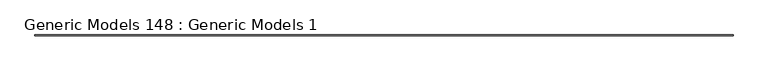
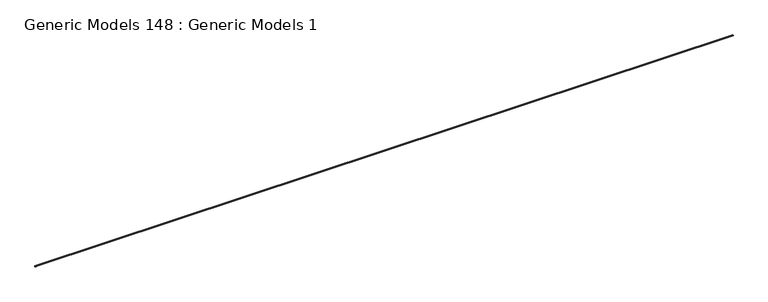
"""IFC4 building model written with IfcOpenShell, lengths in millimetres: proxy geometry, Generic Models 148 : Generic Models 1."""

import ifcopenshell
import ifcopenshell.guid

model = None  # the IFC model being written
_history = None  # IfcOwnerHistory: only IFC2X3 demands one
_inside = {}  # id of a spatial element -> (the spatial element, [elements in it])
_under = {}  # id of a project, library or spatial element -> (it, [spatial elements below it])
_declared = {}  # id of a project -> (the project, [libraries it declares])
_typed = {}  # id of a type object -> (the type object, [elements of that type])
_made_of = {}  # id of a material, layer set ... -> (it, [elements and type objects made of it])


def new_model(schema):
    """Start an empty IFC model of exactly this schema.

    Asked for "IFC4X3", IfcOpenShell would pick the latest addendum, in which some entities
    have other attributes; the version numbers below select the first issue.
    IFC2X3 requires an IfcOwnerHistory on every rooted entity: one is made here for all.
    """
    global model, _history
    if schema == "IFC4X3":
        model = ifcopenshell.file(schema_version=(4, 3, 0, 0))
    else:
        model = ifcopenshell.file(schema=schema)
    _inside.clear()
    _under.clear()
    _declared.clear()
    _typed.clear()
    _made_of.clear()
    _history = None
    if model.schema == "IFC2X3":
        org = make("IfcOrganization", Name="unknown")
        user = make(
            "IfcPersonAndOrganization",
            ThePerson=make("IfcPerson", FamilyName="unknown"),
            TheOrganization=org,
        )
        app = make(
            "IfcApplication",
            ApplicationDeveloper=org,
            Version="unknown",
            ApplicationFullName="unknown",
            ApplicationIdentifier="unknown",
        )
        _history = make(
            "IfcOwnerHistory",
            OwningUser=user,
            OwningApplication=app,
            ChangeAction="ADDED",
            CreationDate=0,
        )
    return model


def make(cls, **values):
    """One entity of the class cls with the attributes given. An attribute that is None is left unset."""
    return model.create_entity(
        cls, **{name: value for name, value in values.items() if value is not None}
    )


def rooted(cls, **values):
    """An entity with a GlobalId (a new one), such as an element, a storey or a relation."""
    return make(cls, GlobalId=ifcopenshell.guid.new(), OwnerHistory=_history, **values)


def si_unit(unit_type, name, prefix=None):
    """IfcSIUnit, for example si_unit("LENGTHUNIT", "METRE", prefix="MILLI")."""
    return make("IfcSIUnit", UnitType=unit_type, Prefix=prefix, Name=name)


def assignment(units):
    """IfcUnitAssignment: the units of a project."""
    return None if units is None else make("IfcUnitAssignment", Units=units)


def point(xyz):
    """IfcCartesianPoint."""
    return None if xyz is None else make("IfcCartesianPoint", Coordinates=xyz)


def direction(xyz):
    """IfcDirection."""
    return None if xyz is None else make("IfcDirection", DirectionRatios=xyz)


def frame(location, z_axis=None, x_axis=None):
    """IfcAxis2Placement3D, a coordinate frame: its origin and axes. An axis left out is left unset."""
    return make(
        "IfcAxis2Placement3D",
        Location=point(location),
        Axis=direction(z_axis),
        RefDirection=direction(x_axis),
    )


def frame_2d(location, x_axis=None):
    """IfcAxis2Placement2D, a coordinate frame in the plane: its origin and x axis."""
    return make(
        "IfcAxis2Placement2D", Location=point(location), RefDirection=direction(x_axis)
    )


def origin():
    """The frame at (0, 0, 0) with its axes left unset."""
    return frame((0.0, 0.0, 0.0))


def place(relative_to, where):
    """IfcLocalPlacement: puts the frame where relative to a parent placement (None: the world)."""
    return make(
        "IfcLocalPlacement", PlacementRelTo=relative_to, RelativePlacement=where
    )


def context(
    kind, dimensions, precision=None, world=None, true_north=None, identifier=None
):
    """IfcGeometricRepresentationContext, for example the 3D "Model" context."""
    return make(
        "IfcGeometricRepresentationContext",
        ContextIdentifier=identifier,
        ContextType=kind,
        CoordinateSpaceDimension=dimensions,
        Precision=precision,
        WorldCoordinateSystem=world,
        TrueNorth=true_north,
    )


def project(units=None, contexts=None):
    """IfcProject with its units and contexts."""
    return rooted(
        "IfcProject",
        Name="project",
        RepresentationContexts=contexts,
        UnitsInContext=assignment(units),
    )


def spatial(cls, under=None, at=None, **own):
    """A site, building, storey or space (cls), placed at a placement, below another one or the project."""
    s = rooted(cls, ObjectPlacement=at, **own)
    if under is not None:
        _under.setdefault(under.id(), (under, []))[1].append(s)
    return s


def polyline(points):
    """IfcPolyline through the points."""
    return make("IfcPolyline", Points=[point(p) for p in points])


def circle_curve(where, radius):
    """IfcCircle in the frame where."""
    return make("IfcCircle", Position=where, Radius=radius)


def trimmed(basis, trim1, trim2, sense, master):
    """IfcTrimmedCurve: the piece of a basis curve between two trims."""
    return make(
        "IfcTrimmedCurve",
        BasisCurve=basis,
        Trim1=trim1,
        Trim2=trim2,
        SenseAgreement=sense,
        MasterRepresentation=master,
    )


def segment(curve, same_sense, transition):
    """IfcCompositeCurveSegment."""
    return make(
        "IfcCompositeCurveSegment",
        Transition=transition,
        SameSense=same_sense,
        ParentCurve=curve,
    )


def composite_curve(segments, self_intersect=None):
    """IfcCompositeCurve: segments joined end to end."""
    return make("IfcCompositeCurve", Segments=segments, SelfIntersect=self_intersect)


def outline(outer, holes=None, kind="AREA"):
    """IfcArbitraryClosedProfileDef: a profile drawn as a closed curve; with holes, ...WithVoids."""
    if holes is None:
        return make("IfcArbitraryClosedProfileDef", ProfileType=kind, OuterCurve=outer)
    return make(
        "IfcArbitraryProfileDefWithVoids",
        ProfileType=kind,
        OuterCurve=outer,
        InnerCurves=holes,
    )


def extrude(swept, where, along, depth):
    """IfcExtrudedAreaSolid: the profile swept, set in the frame where, extruded along a direction by depth."""
    return make(
        "IfcExtrudedAreaSolid",
        SweptArea=swept,
        Position=where,
        ExtrudedDirection=direction(along),
        Depth=depth,
    )


def shape(context_of_items, identifier, shape_type, items):
    """IfcShapeRepresentation: the items that make up one representation, for example the "Body"."""
    return make(
        "IfcShapeRepresentation",
        ContextOfItems=context_of_items,
        RepresentationIdentifier=identifier,
        RepresentationType=shape_type,
        Items=items,
    )


def source(mapping_origin, context_of_items, identifier, shape_type, items):
    """IfcRepresentationMap: a shape defined once, which mapped items show again and again."""
    return make(
        "IfcRepresentationMap",
        MappingOrigin=mapping_origin,
        MappedRepresentation=shape(context_of_items, identifier, shape_type, items),
    )


def transform(
    local_origin,
    x_axis=None,
    y_axis=None,
    z_axis=None,
    scale=None,
    scale2=None,
    scale3=None,
    uniform=True,
):
    """IfcCartesianTransformationOperator3D, or its non-uniform kind. x_axis, y_axis, z_axis: its Axis1, 2, 3."""
    if uniform:
        return make(
            "IfcCartesianTransformationOperator3D",
            Axis1=direction(x_axis),
            Axis2=direction(y_axis),
            LocalOrigin=point(local_origin),
            Scale=scale,
            Axis3=direction(z_axis),
        )
    return make(
        "IfcCartesianTransformationOperator3DnonUniform",
        Axis1=direction(x_axis),
        Axis2=direction(y_axis),
        LocalOrigin=point(local_origin),
        Scale=scale,
        Axis3=direction(z_axis),
        Scale2=scale2,
        Scale3=scale3,
    )


def mapped(mapping_source, mapping_target):
    """IfcMappedItem: shows the shape of a source again, moved by a transform."""
    return make(
        "IfcMappedItem", MappingSource=mapping_source, MappingTarget=mapping_target
    )


def made_of(thing, what):
    """Note that an element or type object is made of a material, layer set ...; save() writes the relation."""
    if what is not None:
        _made_of.setdefault(what.id(), (what, []))[1].append(thing)
    return thing


def element(
    cls,
    number,
    at=None,
    inside=None,
    cuts=None,
    type_object=None,
    material=None,
    context=None,
    identifier="Body",
    shape_type=None,
    held_by="IfcProductDefinitionShape",
    body=None,
    shapes=None,
    **own,
):
    """One element of the class cls, such as IfcWall. Its Tag is "e" and its number.

    at: its placement. inside: the storey or other place that contains it. cuts: it is an
    opening in that element (IfcRelVoidsElement). A single representation is given by context,
    identifier, shape_type and body (its items); several are given by shapes. held_by: the class
    of the entity that holds the representations. save() writes the other relations.
    """
    e = rooted(cls, Tag="e%d" % number, ObjectPlacement=at, **own)
    if body is not None:
        shapes = [shape(context, identifier, shape_type, body)]
    if shapes is not None:
        e.Representation = make(held_by, Representations=shapes)
    if inside is not None:
        _inside.setdefault(inside.id(), (inside, []))[1].append(e)
    if cuts is not None:
        rooted(
            "IfcRelVoidsElement", RelatingBuildingElement=cuts, RelatedOpeningElement=e
        )
    if type_object is not None:
        _typed.setdefault(type_object.id(), (type_object, []))[1].append(e)
    return made_of(e, material)


def aggregate(whole, parts):
    """IfcRelAggregates: a whole, such as a stair, and the parts it consists of."""
    return rooted("IfcRelAggregates", RelatingObject=whole, RelatedObjects=parts)


def save(model, path):
    """Write the relations noted so far, then the file.

    IfcRelAggregates (storeys below a building ...), IfcRelContainedInSpatialStructure (elements
    in a storey), IfcRelDefinesByType, IfcRelAssociatesMaterial and IfcRelDeclares: one each for
    every whole, place, type object, material and project.
    """
    for whole, parts in _under.values():
        aggregate(whole, parts)
    for where, things in _inside.values():
        rooted(
            "IfcRelContainedInSpatialStructure",
            RelatedElements=things,
            RelatingStructure=where,
        )
    for kind, things in _typed.values():
        rooted("IfcRelDefinesByType", RelatedObjects=things, RelatingType=kind)
    for what, things in _made_of.values():
        rooted("IfcRelAssociatesMaterial", RelatedObjects=things, RelatingMaterial=what)
    for by, libraries in _declared.values():
        rooted("IfcRelDeclares", RelatingContext=by, RelatedDefinitions=libraries)
    model.write(path)


def generic_models_148_generic_models_1_1e1312a9(model_context):
    return source(origin(), model_context, "Body", "SweptSolid", [
        extrude(outline(composite_curve([segment(trimmed(circle_curve(frame_2d((7062.6754549, 123920.3246075)), 8.620055), [point((7056.3254549, 123914.4951265))], [point((7069.0254549, 123914.4951265))], True, "CARTESIAN"), True, "CONTINUOUS"), segment(polyline([(7069.0254549, 123914.4951265), (7069.0254549, 123904.9701265)]), True, "CONTINUOUS"), segment(trimmed(circle_curve(frame_2d((7062.6754549, 123910.7996075)), 8.620055), [point((7069.0254549, 123904.9701265))], [point((7056.3254549, 123904.9701265))], False, "CARTESIAN"), True, "CONTINUOUS"), segment(polyline([(7056.3254549, 123904.9701265), (7056.3254549, 123914.4951265)]), True, "CONTINUOUS")], self_intersect=False)), frame((20644.6159513, 0.0, 0.0), z_axis=(1.0, 0.0, 0.0), x_axis=(0.0, 1.0, 0.0)), (0.0, 0.0, 1.0), 12344.4),
    ])


if __name__ == "__main__":
    model = new_model("IFC4")
    model_context = context("Model", 3, world=origin())
    ifc_project = project(units=[si_unit("LENGTHUNIT", "METRE", prefix="MILLI")], contexts=[model_context])
    site = spatial("IfcSite", under=ifc_project)
    building = spatial("IfcBuilding", under=site)
    placement = place(None, origin())
    generic_models_148_generic_models_1_shape = generic_models_148_generic_models_1_1e1312a9(model_context)
    element("IfcBuildingElementProxy", 1, Name="Generic Models 148 : Generic Models 1", ObjectType="Generic Models 148 : Generic Models 1", at=placement, inside=building, context=model_context, shape_type="MappedRepresentation", body=[
        mapped(generic_models_148_generic_models_1_shape, transform((0.0, 0.0, 0.0), x_axis=(1.0, 0.0, 0.0), y_axis=(0.0, 1.0, 0.0), z_axis=(0.0, 0.0, 1.0))),
    ])
    save(model, "model.ifc")

# Revit data of these elements
# Element 1 (IfcBuildingElementProxy, "Generic Models 148 : Generic Models 1")
#   Materials on its faces: "_SEALANT JOINT"
# Materials
#   "_SEALANT JOINT": class "Generic", colour RGB 190 220 196, transparency 0, Cost = 0
